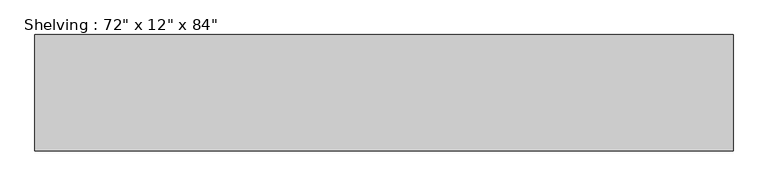
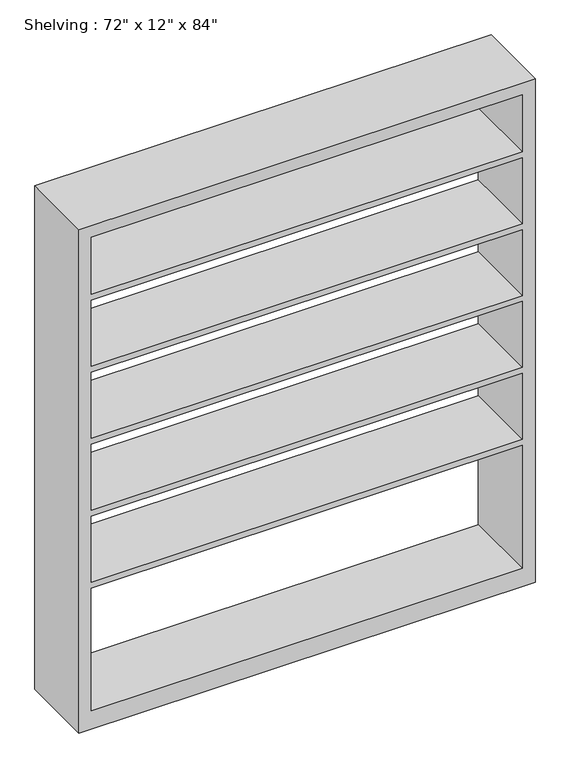
"""IFC4 building model written with IfcOpenShell, lengths in millimetres: furniture geometry."""

from ifc_helpers import new_model, si_unit, frame, origin, place, context, project, spatial, polyline, outline, extrude, source, transform, mapped, element, save


def furniture_6f8441ab(model_context):
    return source(origin(), model_context, "Body", "SweptSolid", [
        extrude(outline(polyline([(0.0, 914.4), (2133.6, 914.4), (2133.6, -914.4), (0.0, -914.4), (0.0, 914.4)]), holes=[polyline([(2082.8, 863.6), (1841.5, 863.6), (1841.5, -863.6), (2082.8, -863.6), (2082.8, 863.6)]), polyline([(76.2, 863.6), (76.2, -863.6), (596.9, -863.6), (596.9, 863.6), (76.2, 863.6)]), polyline([(1231.9, -863.6), (1511.3, -863.6), (1511.3, 863.6), (1231.9, 863.6), (1231.9, -863.6)]), polyline([(1816.1, 863.6), (1536.7, 863.6), (1536.7, -863.6), (1816.1, -863.6), (1816.1, 863.6)]), polyline([(1206.5, 863.6), (927.1, 863.6), (927.1, -863.6), (1206.5, -863.6), (1206.5, 863.6)]), polyline([(901.7, 863.6), (622.3, 863.6), (622.3, -863.6), (901.7, -863.6), (901.7, 863.6)])]), frame((0.0, -457.2, 0.0), z_axis=(0.0, 1.0, 0.0), x_axis=(0.0, 0.0, 1.0)), (0.0, 0.0, 1.0), 304.8),
    ])


if __name__ == "__main__":
    model = new_model("IFC4")
    model_context = context("Model", 3, world=origin())
    ifc_project = project(units=[si_unit("LENGTHUNIT", "METRE", prefix="MILLI")], contexts=[model_context])
    site = spatial("IfcSite", under=ifc_project)
    building = spatial("IfcBuilding", under=site)
    placement = place(None, origin())
    furniture_shape = furniture_6f8441ab(model_context)
    element("IfcFurniture", 1, ObjectType="Shelving : 72\" x 12\" x 84\"", at=placement, inside=building, context=model_context, shape_type="MappedRepresentation", body=[
        mapped(furniture_shape, transform((0.0, 0.0, 0.0), x_axis=(1.0, 0.0, 0.0), y_axis=(0.0, 1.0, 0.0), z_axis=(0.0, 0.0, 1.0))),
    ])
    save(model, "model.ifc")

# Revit data of these elements
# Type "Shelving : 72\" x 12\" x 84\""
#   Assembly Code = "E2020200"
#   Depth = 1' - 0"
#   Height = 7' - 0"
#   Width = 6' - 0"
#   Shelving Unit Material = Wood - Birch
# Element 1 (IfcFurniture, "Shelving : 72\" x 12\" x 84\"")
#   Materials on its faces: "Wood - Birch"
# Materials
#   "Wood - Birch": class "Wood", colour RGB 185 153 119, transparency 0, Comments = "Rendering appearance not upgraded Rendering appearance not upgraded "
